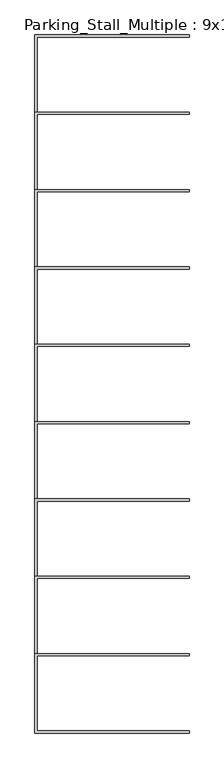
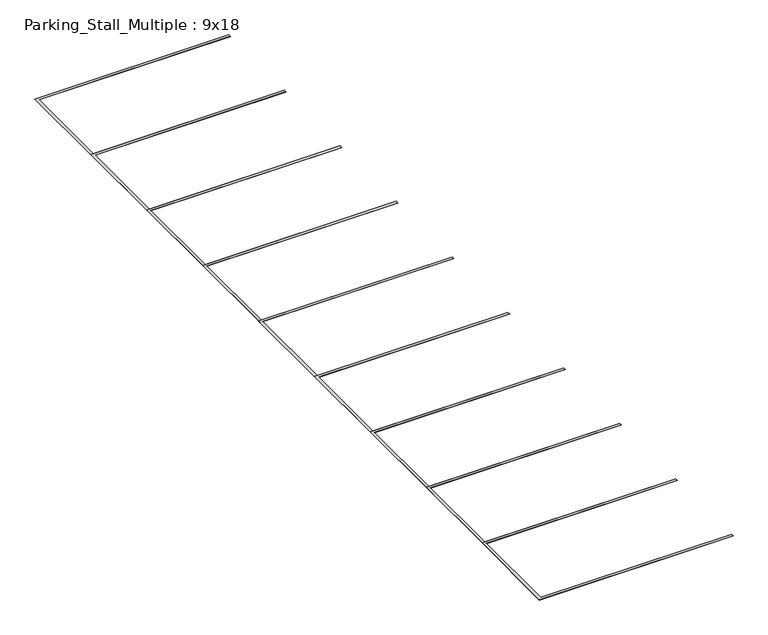
"""IFC4 building model written with IfcOpenShell, lengths in millimetres: proxy geometry, Parking_Stall_Multiple : 9x18."""

import ifcopenshell
import ifcopenshell.guid

model = None  # the IFC model being written
_history = None  # IfcOwnerHistory: only IFC2X3 demands one
_inside = {}  # id of a spatial element -> (the spatial element, [elements in it])
_under = {}  # id of a project, library or spatial element -> (it, [spatial elements below it])
_declared = {}  # id of a project -> (the project, [libraries it declares])
_typed = {}  # id of a type object -> (the type object, [elements of that type])
_made_of = {}  # id of a material, layer set ... -> (it, [elements and type objects made of it])


def new_model(schema):
    """Start an empty IFC model of exactly this schema.

    Asked for "IFC4X3", IfcOpenShell would pick the latest addendum, in which some entities
    have other attributes; the version numbers below select the first issue.
    IFC2X3 requires an IfcOwnerHistory on every rooted entity: one is made here for all.
    """
    global model, _history
    if schema == "IFC4X3":
        model = ifcopenshell.file(schema_version=(4, 3, 0, 0))
    else:
        model = ifcopenshell.file(schema=schema)
    _inside.clear()
    _under.clear()
    _declared.clear()
    _typed.clear()
    _made_of.clear()
    _history = None
    if model.schema == "IFC2X3":
        org = make("IfcOrganization", Name="unknown")
        user = make(
            "IfcPersonAndOrganization",
            ThePerson=make("IfcPerson", FamilyName="unknown"),
            TheOrganization=org,
        )
        app = make(
            "IfcApplication",
            ApplicationDeveloper=org,
            Version="unknown",
            ApplicationFullName="unknown",
            ApplicationIdentifier="unknown",
        )
        _history = make(
            "IfcOwnerHistory",
            OwningUser=user,
            OwningApplication=app,
            ChangeAction="ADDED",
            CreationDate=0,
        )
    return model


def make(cls, **values):
    """One entity of the class cls with the attributes given. An attribute that is None is left unset."""
    return model.create_entity(
        cls, **{name: value for name, value in values.items() if value is not None}
    )


def rooted(cls, **values):
    """An entity with a GlobalId (a new one), such as an element, a storey or a relation."""
    return make(cls, GlobalId=ifcopenshell.guid.new(), OwnerHistory=_history, **values)


def si_unit(unit_type, name, prefix=None):
    """IfcSIUnit, for example si_unit("LENGTHUNIT", "METRE", prefix="MILLI")."""
    return make("IfcSIUnit", UnitType=unit_type, Prefix=prefix, Name=name)


def assignment(units):
    """IfcUnitAssignment: the units of a project."""
    return None if units is None else make("IfcUnitAssignment", Units=units)


def point(xyz):
    """IfcCartesianPoint."""
    return None if xyz is None else make("IfcCartesianPoint", Coordinates=xyz)


def direction(xyz):
    """IfcDirection."""
    return None if xyz is None else make("IfcDirection", DirectionRatios=xyz)


def frame(location, z_axis=None, x_axis=None):
    """IfcAxis2Placement3D, a coordinate frame: its origin and axes. An axis left out is left unset."""
    return make(
        "IfcAxis2Placement3D",
        Location=point(location),
        Axis=direction(z_axis),
        RefDirection=direction(x_axis),
    )


def origin():
    """The frame at (0, 0, 0) with its axes left unset."""
    return frame((0.0, 0.0, 0.0))


def origin_with_axes():
    """The frame at (0, 0, 0) with the z axis (0, 0, 1) and the x axis (1, 0, 0) written out."""
    return frame((0.0, 0.0, 0.0), z_axis=(0.0, 0.0, 1.0), x_axis=(1.0, 0.0, 0.0))


def place(relative_to, where):
    """IfcLocalPlacement: puts the frame where relative to a parent placement (None: the world)."""
    return make(
        "IfcLocalPlacement", PlacementRelTo=relative_to, RelativePlacement=where
    )


def context(
    kind, dimensions, precision=None, world=None, true_north=None, identifier=None
):
    """IfcGeometricRepresentationContext, for example the 3D "Model" context."""
    return make(
        "IfcGeometricRepresentationContext",
        ContextIdentifier=identifier,
        ContextType=kind,
        CoordinateSpaceDimension=dimensions,
        Precision=precision,
        WorldCoordinateSystem=world,
        TrueNorth=true_north,
    )


def project(units=None, contexts=None):
    """IfcProject with its units and contexts."""
    return rooted(
        "IfcProject",
        Name="project",
        RepresentationContexts=contexts,
        UnitsInContext=assignment(units),
    )


def spatial(cls, under=None, at=None, **own):
    """A site, building, storey or space (cls), placed at a placement, below another one or the project."""
    s = rooted(cls, ObjectPlacement=at, **own)
    if under is not None:
        _under.setdefault(under.id(), (under, []))[1].append(s)
    return s


def polyline(points):
    """IfcPolyline through the points."""
    return make("IfcPolyline", Points=[point(p) for p in points])


def outline(outer, holes=None, kind="AREA"):
    """IfcArbitraryClosedProfileDef: a profile drawn as a closed curve; with holes, ...WithVoids."""
    if holes is None:
        return make("IfcArbitraryClosedProfileDef", ProfileType=kind, OuterCurve=outer)
    return make(
        "IfcArbitraryProfileDefWithVoids",
        ProfileType=kind,
        OuterCurve=outer,
        InnerCurves=holes,
    )


def extrude(swept, where, along, depth):
    """IfcExtrudedAreaSolid: the profile swept, set in the frame where, extruded along a direction by depth."""
    return make(
        "IfcExtrudedAreaSolid",
        SweptArea=swept,
        Position=where,
        ExtrudedDirection=direction(along),
        Depth=depth,
    )


def shape(context_of_items, identifier, shape_type, items):
    """IfcShapeRepresentation: the items that make up one representation, for example the "Body"."""
    return make(
        "IfcShapeRepresentation",
        ContextOfItems=context_of_items,
        RepresentationIdentifier=identifier,
        RepresentationType=shape_type,
        Items=items,
    )


def source(mapping_origin, context_of_items, identifier, shape_type, items):
    """IfcRepresentationMap: a shape defined once, which mapped items show again and again."""
    return make(
        "IfcRepresentationMap",
        MappingOrigin=mapping_origin,
        MappedRepresentation=shape(context_of_items, identifier, shape_type, items),
    )


def transform(
    local_origin,
    x_axis=None,
    y_axis=None,
    z_axis=None,
    scale=None,
    scale2=None,
    scale3=None,
    uniform=True,
):
    """IfcCartesianTransformationOperator3D, or its non-uniform kind. x_axis, y_axis, z_axis: its Axis1, 2, 3."""
    if uniform:
        return make(
            "IfcCartesianTransformationOperator3D",
            Axis1=direction(x_axis),
            Axis2=direction(y_axis),
            LocalOrigin=point(local_origin),
            Scale=scale,
            Axis3=direction(z_axis),
        )
    return make(
        "IfcCartesianTransformationOperator3DnonUniform",
        Axis1=direction(x_axis),
        Axis2=direction(y_axis),
        LocalOrigin=point(local_origin),
        Scale=scale,
        Axis3=direction(z_axis),
        Scale2=scale2,
        Scale3=scale3,
    )


def mapped(mapping_source, mapping_target):
    """IfcMappedItem: shows the shape of a source again, moved by a transform."""
    return make(
        "IfcMappedItem", MappingSource=mapping_source, MappingTarget=mapping_target
    )


def made_of(thing, what):
    """Note that an element or type object is made of a material, layer set ...; save() writes the relation."""
    if what is not None:
        _made_of.setdefault(what.id(), (what, []))[1].append(thing)
    return thing


def element(
    cls,
    number,
    at=None,
    inside=None,
    cuts=None,
    type_object=None,
    material=None,
    context=None,
    identifier="Body",
    shape_type=None,
    held_by="IfcProductDefinitionShape",
    body=None,
    shapes=None,
    **own,
):
    """One element of the class cls, such as IfcWall. Its Tag is "e" and its number.

    at: its placement. inside: the storey or other place that contains it. cuts: it is an
    opening in that element (IfcRelVoidsElement). A single representation is given by context,
    identifier, shape_type and body (its items); several are given by shapes. held_by: the class
    of the entity that holds the representations. save() writes the other relations.
    """
    e = rooted(cls, Tag="e%d" % number, ObjectPlacement=at, **own)
    if body is not None:
        shapes = [shape(context, identifier, shape_type, body)]
    if shapes is not None:
        e.Representation = make(held_by, Representations=shapes)
    if inside is not None:
        _inside.setdefault(inside.id(), (inside, []))[1].append(e)
    if cuts is not None:
        rooted(
            "IfcRelVoidsElement", RelatingBuildingElement=cuts, RelatedOpeningElement=e
        )
    if type_object is not None:
        _typed.setdefault(type_object.id(), (type_object, []))[1].append(e)
    return made_of(e, material)


def aggregate(whole, parts):
    """IfcRelAggregates: a whole, such as a stair, and the parts it consists of."""
    return rooted("IfcRelAggregates", RelatingObject=whole, RelatedObjects=parts)


def save(model, path):
    """Write the relations noted so far, then the file.

    IfcRelAggregates (storeys below a building ...), IfcRelContainedInSpatialStructure (elements
    in a storey), IfcRelDefinesByType, IfcRelAssociatesMaterial and IfcRelDeclares: one each for
    every whole, place, type object, material and project.
    """
    for whole, parts in _under.values():
        aggregate(whole, parts)
    for where, things in _inside.values():
        rooted(
            "IfcRelContainedInSpatialStructure",
            RelatedElements=things,
            RelatingStructure=where,
        )
    for kind, things in _typed.values():
        rooted("IfcRelDefinesByType", RelatedObjects=things, RelatingType=kind)
    for what, things in _made_of.values():
        rooted("IfcRelAssociatesMaterial", RelatedObjects=things, RelatingMaterial=what)
    for by, libraries in _declared.values():
        rooted("IfcRelDeclares", RelatingContext=by, RelatedDefinitions=libraries)
    model.write(path)


def parking_stall_multiple_9x18_3a9ea78d(model_context):
    return source(origin(), model_context, "Body", "SweptSolid", [
        extrude(outline(polyline([(5486.4, -21945.6), (5486.4, -22021.8), (76.2, -22021.8), (76.2, -24688.8), (5486.4, -24688.8), (5486.4, -24765.0), (0.0, -24765.0), (0.0, -21945.6), (5486.4, -21945.6)])), origin_with_axes(), (0.0, 0.0, 1.0), 6.35),
        extrude(outline(polyline([(5486.4, -19202.4), (5486.4, -19278.6), (76.2, -19278.6), (76.2, -21945.6), (5486.4, -21945.6), (5486.4, -22021.8), (0.0, -22021.8), (0.0, -19202.4), (5486.4, -19202.4)])), origin_with_axes(), (0.0, 0.0, 1.0), 6.35),
        extrude(outline(polyline([(5486.4, -16459.2), (5486.4, -16535.4), (76.2, -16535.4), (76.2, -19202.4), (5486.4, -19202.4), (5486.4, -19278.6), (0.0, -19278.6), (0.0, -16459.2), (5486.4, -16459.2)])), origin_with_axes(), (0.0, 0.0, 1.0), 6.35),
        extrude(outline(polyline([(5486.4, -13716.0), (5486.4, -13792.2), (76.2, -13792.2), (76.2, -16459.2), (5486.4, -16459.2), (5486.4, -16535.4), (0.0, -16535.4), (0.0, -13716.0), (5486.4, -13716.0)])), origin_with_axes(), (0.0, 0.0, 1.0), 6.35),
        extrude(outline(polyline([(5486.4, -10972.8), (5486.4, -11049.0), (76.2, -11049.0), (76.2, -13716.0), (5486.4, -13716.0), (5486.4, -13792.2), (0.0, -13792.2), (0.0, -10972.8), (5486.4, -10972.8)])), origin_with_axes(), (0.0, 0.0, 1.0), 6.35),
        extrude(outline(polyline([(5486.4, -8229.6), (5486.4, -8305.8), (76.2, -8305.8), (76.2, -10972.8), (5486.4, -10972.8), (5486.4, -11049.0), (0.0, -11049.0), (0.0, -8229.6), (5486.4, -8229.6)])), origin_with_axes(), (0.0, 0.0, 1.0), 6.35),
        extrude(outline(polyline([(5486.4, -5486.4), (5486.4, -5562.6), (76.2, -5562.6), (76.2, -8229.6), (5486.4, -8229.6), (5486.4, -8305.8), (0.0, -8305.8), (0.0, -5486.4), (5486.4, -5486.4)])), origin_with_axes(), (0.0, 0.0, 1.0), 6.35),
        extrude(outline(polyline([(5486.4, -2743.2), (5486.4, -2819.4), (76.2, -2819.4), (76.2, -5486.4), (5486.4, -5486.4), (5486.4, -5562.6), (0.0, -5562.6), (0.0, -2743.2), (5486.4, -2743.2)])), origin_with_axes(), (0.0, 0.0, 1.0), 6.35),
        extrude(outline(polyline([(5486.4, 0.0), (5486.4, -76.2), (76.2, -76.2), (76.2, -2743.2), (5486.4, -2743.2), (5486.4, -2819.4), (0.0, -2819.4), (0.0, 0.0), (5486.4, 0.0)])), origin_with_axes(), (0.0, 0.0, 1.0), 6.35),
    ])


if __name__ == "__main__":
    model = new_model("IFC4")
    model_context = context("Model", 3, world=origin())
    ifc_project = project(units=[si_unit("LENGTHUNIT", "METRE", prefix="MILLI")], contexts=[model_context])
    site = spatial("IfcSite", under=ifc_project)
    building = spatial("IfcBuilding", under=site)
    placement = place(None, origin())
    parking_stall_multiple_9x18_shape = parking_stall_multiple_9x18_3a9ea78d(model_context)
    element("IfcBuildingElementProxy", 1, Name="Parking_Stall_Multiple : 9x18", ObjectType="Parking_Stall_Multiple : 9x18", at=placement, inside=building, context=model_context, shape_type="MappedRepresentation", body=[
        mapped(parking_stall_multiple_9x18_shape, transform((0.0, 0.0, 0.0), x_axis=(1.0, 0.0, 0.0), y_axis=(0.0, 1.0, 0.0), z_axis=(0.0, 0.0, 1.0))),
    ])
    save(model, "model.ifc")

# Revit data of these elements
# Type "Parking_Stall_Multiple : 9x18"
#   Parking_Width_M = 9' - 0"
#   Parking_Run_Length [instance default] = 65' - 0"
#   Parking_Line_Width = 0' - 3"
#   Parking_Length_M = 18' - 0"
#   Single_Parking_Visibility [instance default] = no
#   Parking_ADA_Symbol = no
#   ParkingUnitsArray [instance default] = 7
#   ParkingUnits [instance default] = 7
#   Multiple_Parking_Visibility [instance default] = yes
#   Parking_Line_Material = none
# Element 1 (IfcBuildingElementProxy, "Parking_Stall_Multiple : 9x18")
#   Parking_Run_Length = 81' - 3"
#   ParkingUnitsArray = 9
#   ParkingUnits = 9
